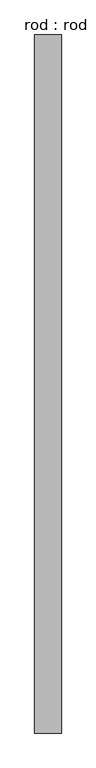
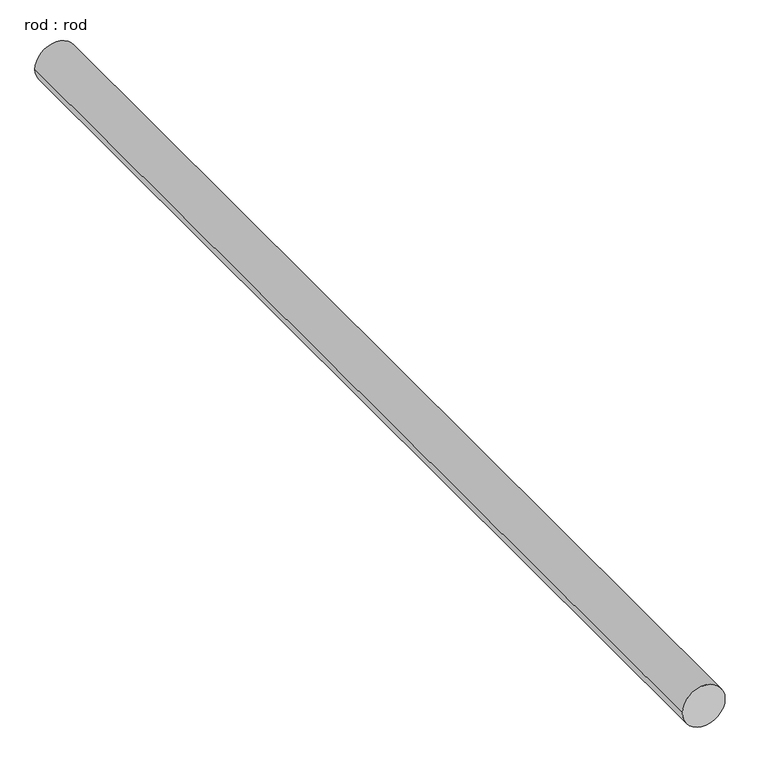
"""IFC4 building model written with IfcOpenShell, lengths in millimetres: proxy geometry, rod : rod."""

from ifc_helpers import new_model, si_unit, point, frame, frame_2d, origin, place, context, project, spatial, circle_curve, trimmed, segment, composite_curve, outline, extrude, source, transform, mapped, element, save


def rod_rod_d1816047(model_context):
    return source(origin(), model_context, "Body", "SweptSolid", [
        extrude(outline(composite_curve([segment(trimmed(circle_curve(frame_2d((0.0108462, 0.0)), 200.0), [point((0.0108462, 200.0))], [point((0.0108462, -200.0))], False, "CARTESIAN"), True, "CONTINUOUS"), segment(trimmed(circle_curve(frame_2d((0.0108462, 0.0)), 200.0), [point((0.0108462, -200.0))], [point((0.0108462, 200.0))], False, "CARTESIAN"), True, "CONTINUOUS")], self_intersect=False)), frame((0.0, -1157.2713847, 0.0), z_axis=(0.0, 1.0, 0.0), x_axis=(0.0, 0.0, 1.0)), (0.0, 0.0, 1.0), 10500.0),
    ])


if __name__ == "__main__":
    model = new_model("IFC4")
    model_context = context("Model", 3, world=origin())
    ifc_project = project(units=[si_unit("LENGTHUNIT", "METRE", prefix="MILLI")], contexts=[model_context])
    site = spatial("IfcSite", under=ifc_project)
    building = spatial("IfcBuilding", under=site)
    placement = place(None, origin())
    rod_rod_shape = rod_rod_d1816047(model_context)
    element("IfcBuildingElementProxy", 1, Name="rod : rod", ObjectType="rod : rod", at=placement, inside=building, context=model_context, shape_type="MappedRepresentation", body=[
        mapped(rod_rod_shape, transform((0.0, 0.0, 0.0), x_axis=(1.0, 0.0, 0.0), y_axis=(0.0, 1.0, 0.0), z_axis=(0.0, 0.0, 1.0))),
    ])
    save(model, "model.ifc")

# Revit data of these elements
# Type "rod : rod"
#   Default Elevation = 0
